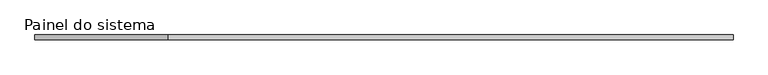
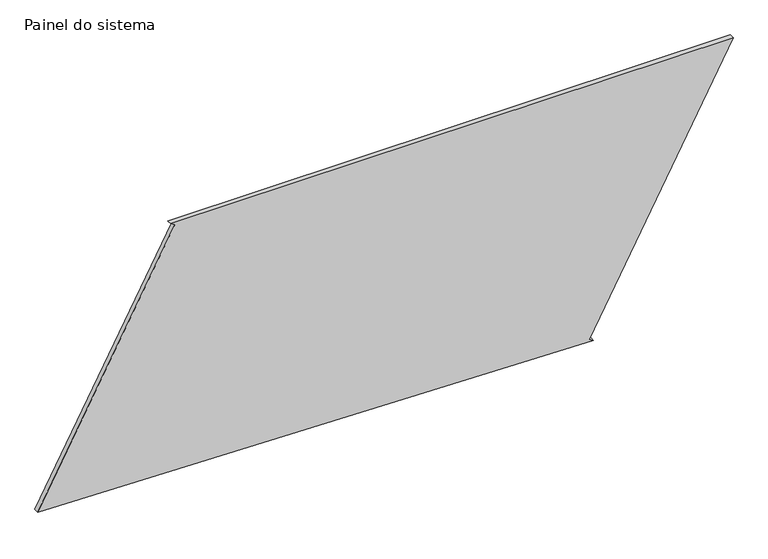
"""IFC4 building model written with IfcOpenShell, lengths in millimetres: plate geometry, Painel do sistema : Envidraçado."""

from ifc_helpers import new_model, si_unit, frame, origin, place, context, project, spatial, polyline, outline, extrude, source, transform, mapped, element, save


def painel_do_sistema_5a387b35(model_context):
    return source(origin(), model_context, "Body", "SweptSolid", [
        extrude(outline(polyline([(0.0, 1068.6588747), (11.7958757, 1046.6167034), (1393.6224162, 1786.1016572), (1393.6224162, -1103.3924162), (1381.8265406, -1081.3502448), (64.9042677, -1786.1016572), (0.0, 1068.6588747)])), frame((0.0, 24.5, 0.0), z_axis=(0.0, 1.0, 0.0), x_axis=(0.0, 0.0, 1.0)), (0.0, 0.0, 1.0), 25.0),
    ])


if __name__ == "__main__":
    model = new_model("IFC4")
    model_context = context("Model", 3, world=origin())
    ifc_project = project(units=[si_unit("LENGTHUNIT", "METRE", prefix="MILLI")], contexts=[model_context])
    site = spatial("IfcSite", under=ifc_project)
    building = spatial("IfcBuilding", under=site)
    placement = place(None, origin())
    painel_do_sistema_shape = painel_do_sistema_5a387b35(model_context)
    element("IfcPlate", 1, ObjectType="Painel do sistema : Envidraçado", at=placement, inside=building, context=model_context, shape_type="MappedRepresentation", body=[
        mapped(painel_do_sistema_shape, transform((0.0, 0.0, 0.0), x_axis=(1.0, 0.0, 0.0), y_axis=(0.0, 1.0, 0.0), z_axis=(0.0, 0.0, 1.0))),
    ])
    save(model, "model.ifc")

# Revit data of these elements
# Type "Painel do sistema : Envidraçado"
#   Construction Type Id = "GSP4R"
#   Analytic Construction = "Vidraça única Pilkington 1/8 pol"
#   Visual Light Transmittance = 0.9
#   Solar Heat Gain Coefficient = 0.86
#   Heat Transfer Coefficient (U) = 6.7069 W/(m²·K)
# Element 1 (IfcPlate, "Painel do sistema : Envidraçado")
#   Materials on its faces: "Vidro"
# Materials
#   "Vidro": class "Vidro", colour RGB 0 128 192, transparency 0.9, Description = "Vidro de sílica", Cost = 0
